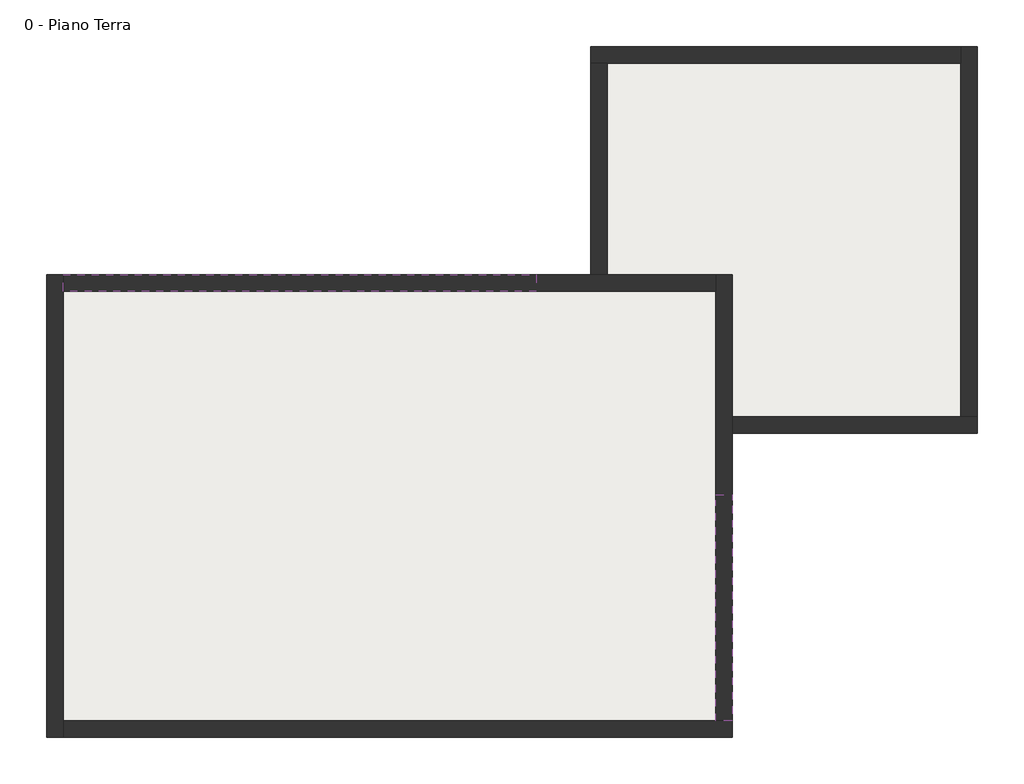
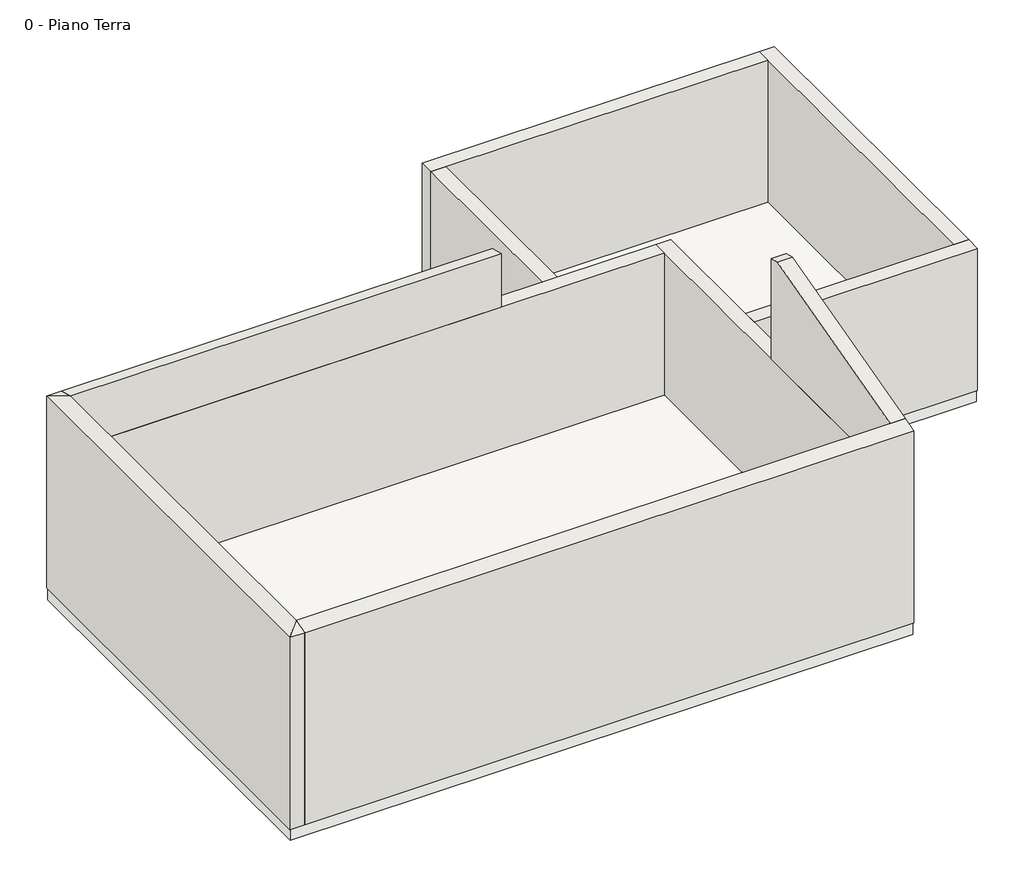
# One storey: 10 walls, 2 slabs.
"""IFC4 building model written with IfcOpenShell, lengths in millimetres."""

from ifc_helpers import new_model, si_unit, frame, origin, origin_with_axes, place, context, project, spatial, polyline, outline, extrude, faceted_brep, element, save

model = new_model("IFC4")

# Units and contexts
model_context = context("Model", 3, world=origin())
ifc_project = project(units=[si_unit("LENGTHUNIT", "METRE", prefix="MILLI")], contexts=[model_context])

# Site, building, storey
site = spatial("IfcSite", under=ifc_project)
building = spatial("IfcBuilding", under=site)
storey = spatial("IfcBuildingStorey", under=building, Name="0 - Piano Terra", Elevation=0.0)

# Slabs
placement = place(None, origin())
element("IfcSlab", 1, ObjectType="Latero Cementizio - 30 cm", at=placement, inside=storey, context=model_context, shape_type="SweptSolid", body=[
    extrude(outline(polyline([(-16900.292668, 14038.4212472), (-1570.292668, 14038.4212472), (-1570.292668, 3708.4212472), (-16900.292668, 3708.4212472), (-16900.292668, 14038.4212472)])), frame((0.0, 0.0, -300.0), z_axis=(0.0, 0.0, 1.0), x_axis=(1.0, 0.0, 0.0)), (0.0, 0.0, 1.0), 300.0),
])
element("IfcSlab", 2, ObjectType="Latero Cementizio - 30 cm", at=placement, inside=storey, context=model_context, shape_type="SweptSolid", body=[
    extrude(outline(polyline([(3929.707332, 10523.4212472), (-1560.292668, 10523.4212472), (-1560.292668, 14058.4212472), (-4700.292668, 14058.4212472), (-4700.292668, 19153.4212472), (3929.707332, 19153.4212472), (3929.707332, 10523.4212472)])), frame((0.0, 0.0, -300.0), z_axis=(0.0, 0.0, 1.0), x_axis=(1.0, 0.0, 0.0)), (0.0, 0.0, 1.0), 300.0),
])

# Walls
element("IfcWall", 3, ObjectType="37 cm", at=placement, inside=storey, context=model_context, shape_type="Brep", body=[
    faceted_brep([(-16920.292668, 14058.4212472, 5000.0), (-16920.292668, 14058.4212472, 0.0), (-16920.292668, 3688.4212472, 0.0), (-16920.292668, 3688.4212472, 5000.0), (-16550.292668, 14058.4212472, 0.0), (-16550.292668, 14058.4212472, 3700.0), (-16550.292668, 14058.4212472, 5000.0), (-16550.292668, 13688.4212472, 5099.1412012), (-16550.292668, 4058.4212472, 5099.1412012), (-16550.292668, 3688.4212472, 5000.0), (-16550.292668, 3688.4212472, 0.0), (-16550.292668, 4058.4212472, 0.0), (-16550.292668, 13688.4212472, 0.0)], [[[0, 1, 2, 3]], [[4, 5, 6, 7, 8, 9, 10, 11, 12]], [[2, 1, 4, 12, 11, 10]], [[3, 2, 10, 9]], [[0, 6, 5, 4, 1]], [[0, 3, 8, 7]], [[3, 9, 8]], [[7, 6, 0]]]),
])
element("IfcWall", 4, ObjectType="37 cm", at=placement, inside=storey, context=model_context, shape_type="Brep", body=[
    faceted_brep([(-16550.292668, 3688.4212472, 0.0), (-1550.292668, 3688.4212472, 0.0), (-1550.292668, 3688.4212472, 5000.0), (-16550.292668, 3688.4212472, 5000.0), (-16550.292668, 4058.4212472, 0.0), (-16550.292668, 4058.4212472, 5099.1412012), (-1920.292668, 4058.4212472, 5099.1412012), (-1550.292668, 4058.4212472, 5099.1412012), (-1550.292668, 4058.4212472, 3700.0), (-1550.292668, 4058.4212472, 0.0), (-1920.292668, 4058.4212472, 0.0)], [[[0, 1, 2, 3]], [[4, 5, 6, 7, 8, 9, 10]], [[1, 0, 4, 10, 9]], [[0, 3, 5, 4]], [[1, 9, 8, 7, 2]], [[3, 2, 7, 6, 5]]]),
])
element("IfcWall", 5, ObjectType="37 cm", at=placement, inside=storey, context=model_context, shape_type="Brep", body=[
    faceted_brep([(-1550.292668, 4058.4212472, 0.0), (-1550.292668, 10503.4212472, 0.0), (-1550.292668, 10873.4212472, 0.0), (-1550.292668, 14058.4212472, 0.0), (-1550.292668, 14058.4212472, 3700.0), (-1550.292668, 10873.4212472, 3700.0), (-1550.292668, 10503.4212472, 3700.0), (-1550.292668, 9128.4386987, 3700.0), (-1550.292668, 4058.4212472, 3700.0), (-1920.292668, 4058.4212472, 0.0), (-1920.292668, 4058.4212472, 3700.0), (-1920.292668, 9128.4386987, 3700.0), (-1920.292668, 13688.4212472, 3700.0), (-1920.292668, 14058.4212472, 3700.0), (-1920.292668, 14058.4212472, 0.0), (-1920.292668, 13688.4212472, 0.0)], [[[0, 1, 2, 3, 4, 5, 6, 7, 8]], [[9, 10, 11, 12, 13, 14, 15]], [[3, 2, 1, 0, 9, 15, 14]], [[8, 7, 6, 5, 4, 13, 12, 11, 10]], [[0, 8, 10, 9]], [[4, 3, 14, 13]]]),
])
element("IfcWall", 6, ObjectType="37 cm", at=placement, inside=storey, context=model_context, shape_type="Brep", body=[
    faceted_brep([(-1920.292668, 14058.4212472, 0.0), (-4350.292668, 14058.4212472, 0.0), (-4720.292668, 14058.4212472, 0.0), (-16550.292668, 14058.4212472, 0.0), (-16550.292668, 14058.4212472, 3700.0), (-5941.300812, 14058.4212472, 3700.0), (-4720.292668, 14058.4212472, 3700.0), (-4350.292668, 14058.4212472, 3700.0), (-1920.292668, 14058.4212472, 3700.0), (-1920.292668, 13688.4212472, 0.0), (-1920.292668, 13688.4212472, 3700.0), (-5941.300812, 13688.4212472, 3700.0), (-16550.292668, 13688.4212472, 3700.0), (-16550.292668, 13688.4212472, 0.0)], [[[0, 1, 2, 3, 4, 5, 6, 7, 8]], [[9, 10, 11, 12, 13]], [[3, 2, 1, 0, 9, 13]], [[8, 7, 6, 5, 4, 12, 11, 10]], [[4, 3, 13, 12]], [[0, 8, 10, 9]]]),
])
element("IfcWall", 7, ObjectType="37 cm", at=placement, inside=storey, context=model_context, shape_type="Brep", body=[
    faceted_brep([(-1550.292668, 10503.4212472, 0.0), (3949.707332, 10503.4212472, 0.0), (3949.707332, 10503.4212472, 3700.0), (-1550.292668, 10503.4212472, 3700.0), (-1550.292668, 10873.4212472, 0.0), (-1550.292668, 10873.4212472, 3700.0), (3579.707332, 10873.4212472, 3700.0), (3949.707332, 10873.4212472, 3700.0), (3949.707332, 10873.4212472, 0.0), (3579.707332, 10873.4212472, 0.0)], [[[0, 1, 2, 3]], [[4, 5, 6, 7, 8, 9]], [[1, 0, 4, 9, 8]], [[3, 2, 7, 6, 5]], [[0, 3, 5, 4]], [[2, 1, 8, 7]]]),
])
element("IfcWall", 8, ObjectType="37 cm", at=placement, inside=storey, context=model_context, shape_type="Brep", body=[
    faceted_brep([(3949.707332, 10873.4212472, 0.0), (3949.707332, 19173.4212472, 0.0), (3949.707332, 19173.4212472, 3700.0), (3949.707332, 10873.4212472, 3700.0), (3579.707332, 10873.4212472, 0.0), (3579.707332, 10873.4212472, 3700.0), (3579.707332, 18803.4212472, 3700.0), (3579.707332, 19173.4212472, 3700.0), (3579.707332, 19173.4212472, 0.0), (3579.707332, 18803.4212472, 0.0)], [[[0, 1, 2, 3]], [[4, 5, 6, 7, 8, 9]], [[1, 0, 4, 9, 8]], [[3, 2, 7, 6, 5]], [[0, 3, 5, 4]], [[2, 1, 8, 7]]]),
])
element("IfcWall", 9, ObjectType="37 cm", at=placement, inside=storey, context=model_context, shape_type="Brep", body=[
    faceted_brep([(3579.707332, 19173.4212472, 0.0), (-4720.292668, 19173.4212472, 0.0), (-4720.292668, 19173.4212472, 3700.0), (3579.707332, 19173.4212472, 3700.0), (3579.707332, 18803.4212472, 0.0), (3579.707332, 18803.4212472, 3700.0), (-4350.292668, 18803.4212472, 3700.0), (-4720.292668, 18803.4212472, 3700.0), (-4720.292668, 18803.4212472, 0.0), (-4350.292668, 18803.4212472, 0.0)], [[[0, 1, 2, 3]], [[4, 5, 6, 7, 8, 9]], [[1, 0, 4, 9, 8]], [[3, 2, 7, 6, 5]], [[0, 3, 5, 4]], [[2, 1, 8, 7]]]),
])
element("IfcWall", 10, ObjectType="37 cm", at=placement, inside=storey, context=model_context, shape_type="SweptSolid", body=[
    extrude(outline(polyline([(-4720.292668, 14058.4212472), (-4720.292668, 18803.4212472), (-4350.292668, 18803.4212472), (-4350.292668, 14058.4212472), (-4720.292668, 14058.4212472)])), origin_with_axes(), (0.0, 0.0, 1.0), 3700.0),
])
element("IfcWall", 11, ObjectType="37 cm", at=placement, inside=storey, context=model_context, shape_type="SweptSolid", body=[
    extrude(outline(polyline([(4058.4212472, 3700.0), (4058.4212472, 5099.1412012), (8873.4212472, 6389.3165628), (9128.4386987, 6320.9848426), (9128.4386987, 3700.0), (4058.4212472, 3700.0)])), frame((-1920.292668, 0.0, 0.0), z_axis=(1.0, 0.0, 0.0), x_axis=(0.0, 1.0, 0.0)), (0.0, 0.0, 1.0), 370.0),
])
element("IfcWall", 12, ObjectType="37 cm", at=placement, inside=storey, context=model_context, shape_type="SweptSolid", body=[
    extrude(outline(polyline([(14058.4212472, 5000.0), (14058.4212472, 3700.0), (13688.4212472, 3700.0), (13688.4212472, 5099.1412012), (14058.4212472, 5000.0)])), frame((-16550.292668, 0.0, 0.0), z_axis=(1.0, 0.0, 0.0), x_axis=(0.0, 1.0, 0.0)), (0.0, 0.0, 1.0), 10608.9918559),
])

save(model, "model.ifc")

# Revit data of these elements
# Project information
#   Data di consegna del progetto = "Data"
#   Stato del progetto = "Stato"
#   Nome del cliente = "Proprietario"
#   Nome del progetto = "Nome"
#   Numero del progetto = "0001"
# Type "Latero Cementizio - 30 cm"
#   Keynote = "S/3"
#   Function = 0
#   Layers, outside or top first: 0.02 m "Ceramica bianca" (function 4); 0.065 m "Sabbia e Calcestruzzo" (function 2); 0.04 m "Calcestruzzo" (function 1); 0.16 m "Laterizio (2)" (function 1); 0.015 m "Intonaco - Bianco" (function 5)
# Type "37 cm"
#   Keynote = "Mb/3"
#   Layers, outside or top first: 0.02 m "Intonaco esterno" (function 1); 0.08 m "Isolamento" (function 1); 0.25 m "Calcestruzzo Blocchi" (function 1); 0.02 m "Intonaco interno" (function 5)
# Element 1 (IfcSlab, "Latero Cementizio - 30 cm")
#   built-in parameter 1001955 = 3.14159 (stored number, unit not read)
#   Height Offset From Level = 0.00 m
#   Phase Created = Stato di Progetto
#   Materials on its faces: "Intonaco - Bianco", "Ceramica bianca"
# Element 2 (IfcSlab, "Latero Cementizio - 30 cm")
#   Height Offset From Level = 0.00 m
#   Phase Created = Stato di Progetto
#   Materials on its faces: "Intonaco - Bianco", "Ceramica bianca"
# Elements 3, 4 (IfcWall, "37 cm")
#   Top Offset = 0.00 m
#   Base Offset = 0.00 m
#   Unconnected Height = 5.00 m
#   wall height = 5.00 m
#   Phase Created = Stato di Progetto
#   Base Constraint = 0 - Piano Terra
#   Materials on its faces: "Default - Calcestruzzo", "Intonaco interno", "Intonaco esterno"
# Elements 5, 6, 7, 8, 9, 10 (IfcWall, "37 cm")
#   Top Offset = 0.00 m
#   Base Offset = 0.00 m
#   Unconnected Height = 3.70 m
#   wall height = 3.70 m
#   Phase Created = Stato di Progetto
#   Base Constraint = 0 - Piano Terra
#   Materials on its faces: "Default - Calcestruzzo", "Intonaco interno", "Intonaco esterno"
# Elements 11, 12 (IfcWall, "37 cm")
#   built-in parameter 1001111 = 3.70 m
#   Top Offset = 0.00 m
#   Base Offset = 3.70 m
#   Unconnected Height = 1.30 m
#   wall height = 1.30 m
#   Phase Created = Stato di Progetto
#   Base Constraint = 0 - Piano Terra
#   Materials on its faces: "Default - Calcestruzzo", "Intonaco interno", "Intonaco esterno"
# Materials
#   "Ceramica bianca": class "Ceramica", colour RGB 210 210 210, transparency 0, Description = "Finitura interna - Piastrelle di ceramica incollate", Cost = 0
#   "Sabbia e Calcestruzzo": class "Calcestruzzo", colour RGB 127 127 127, transparency 0, Description = "Magrone - Sabbia e cemento", Cost = 0
#   "Calcestruzzo": class "Calcestruzzo", colour RGB 192 192 192, transparency 0, Description = "Calcestruzzo - Cemento Portland", Cost = 0
#   "Laterizio (2)": class "Mattone", colour RGB 255 128 64, transparency 0, Description = "Pignatta h 16 cm", Cost = 0
#   "Intonaco - Bianco": class "Intonaco", colour RGB 249 249 249, transparency 0, Description = "Verniciatura", Cost = 0
#   "Intonaco esterno": class "Intonaco", colour RGB 249 249 249, transparency 0, Description = "Verniciatura", Cost = 0
#   "Isolamento": class "Varie", colour RGB 127 127 127, transparency 0, Description = "Pannello in sughero", Cost = 0
#   "Calcestruzzo Blocchi": class "Calcestruzzo", colour RGB 255 128 0, transparency 0, Description = "Calcestruzzo - Cemento Portland", Cost = 0
#   "Intonaco interno": class "Intonaco", colour RGB 249 249 249, transparency 0, Description = "Verniciatura", Cost = 0
#   "Default - Calcestruzzo": class "Calcestruzzo", colour RGB 192 192 192, transparency 0, Description = "Calcestruzzo", Cost = 0
